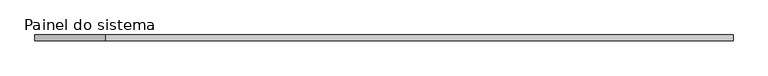
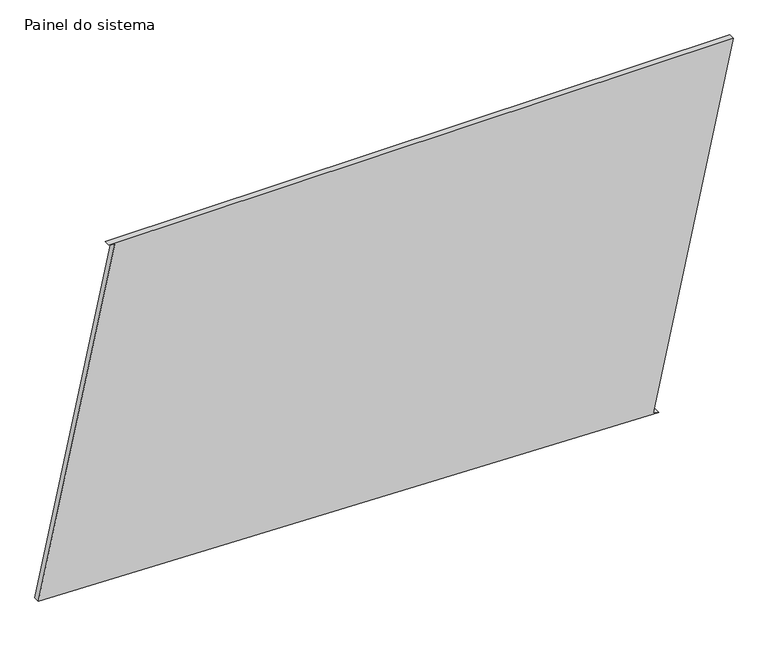
"""IFC4 building model written with IfcOpenShell, lengths in millimetres: plate geometry, Painel do sistema : Envidraçado."""

import ifcopenshell
import ifcopenshell.guid

model = None  # the IFC model being written
_history = None  # IfcOwnerHistory: only IFC2X3 demands one
_inside = {}  # id of a spatial element -> (the spatial element, [elements in it])
_under = {}  # id of a project, library or spatial element -> (it, [spatial elements below it])
_declared = {}  # id of a project -> (the project, [libraries it declares])
_typed = {}  # id of a type object -> (the type object, [elements of that type])
_made_of = {}  # id of a material, layer set ... -> (it, [elements and type objects made of it])


def new_model(schema):
    """Start an empty IFC model of exactly this schema.

    Asked for "IFC4X3", IfcOpenShell would pick the latest addendum, in which some entities
    have other attributes; the version numbers below select the first issue.
    IFC2X3 requires an IfcOwnerHistory on every rooted entity: one is made here for all.
    """
    global model, _history
    if schema == "IFC4X3":
        model = ifcopenshell.file(schema_version=(4, 3, 0, 0))
    else:
        model = ifcopenshell.file(schema=schema)
    _inside.clear()
    _under.clear()
    _declared.clear()
    _typed.clear()
    _made_of.clear()
    _history = None
    if model.schema == "IFC2X3":
        org = make("IfcOrganization", Name="unknown")
        user = make(
            "IfcPersonAndOrganization",
            ThePerson=make("IfcPerson", FamilyName="unknown"),
            TheOrganization=org,
        )
        app = make(
            "IfcApplication",
            ApplicationDeveloper=org,
            Version="unknown",
            ApplicationFullName="unknown",
            ApplicationIdentifier="unknown",
        )
        _history = make(
            "IfcOwnerHistory",
            OwningUser=user,
            OwningApplication=app,
            ChangeAction="ADDED",
            CreationDate=0,
        )
    return model


def make(cls, **values):
    """One entity of the class cls with the attributes given. An attribute that is None is left unset."""
    return model.create_entity(
        cls, **{name: value for name, value in values.items() if value is not None}
    )


def rooted(cls, **values):
    """An entity with a GlobalId (a new one), such as an element, a storey or a relation."""
    return make(cls, GlobalId=ifcopenshell.guid.new(), OwnerHistory=_history, **values)


def si_unit(unit_type, name, prefix=None):
    """IfcSIUnit, for example si_unit("LENGTHUNIT", "METRE", prefix="MILLI")."""
    return make("IfcSIUnit", UnitType=unit_type, Prefix=prefix, Name=name)


def assignment(units):
    """IfcUnitAssignment: the units of a project."""
    return None if units is None else make("IfcUnitAssignment", Units=units)


def point(xyz):
    """IfcCartesianPoint."""
    return None if xyz is None else make("IfcCartesianPoint", Coordinates=xyz)


def direction(xyz):
    """IfcDirection."""
    return None if xyz is None else make("IfcDirection", DirectionRatios=xyz)


def frame(location, z_axis=None, x_axis=None):
    """IfcAxis2Placement3D, a coordinate frame: its origin and axes. An axis left out is left unset."""
    return make(
        "IfcAxis2Placement3D",
        Location=point(location),
        Axis=direction(z_axis),
        RefDirection=direction(x_axis),
    )


def origin():
    """The frame at (0, 0, 0) with its axes left unset."""
    return frame((0.0, 0.0, 0.0))


def place(relative_to, where):
    """IfcLocalPlacement: puts the frame where relative to a parent placement (None: the world)."""
    return make(
        "IfcLocalPlacement", PlacementRelTo=relative_to, RelativePlacement=where
    )


def context(
    kind, dimensions, precision=None, world=None, true_north=None, identifier=None
):
    """IfcGeometricRepresentationContext, for example the 3D "Model" context."""
    return make(
        "IfcGeometricRepresentationContext",
        ContextIdentifier=identifier,
        ContextType=kind,
        CoordinateSpaceDimension=dimensions,
        Precision=precision,
        WorldCoordinateSystem=world,
        TrueNorth=true_north,
    )


def project(units=None, contexts=None):
    """IfcProject with its units and contexts."""
    return rooted(
        "IfcProject",
        Name="project",
        RepresentationContexts=contexts,
        UnitsInContext=assignment(units),
    )


def spatial(cls, under=None, at=None, **own):
    """A site, building, storey or space (cls), placed at a placement, below another one or the project."""
    s = rooted(cls, ObjectPlacement=at, **own)
    if under is not None:
        _under.setdefault(under.id(), (under, []))[1].append(s)
    return s


def polyline(points):
    """IfcPolyline through the points."""
    return make("IfcPolyline", Points=[point(p) for p in points])


def outline(outer, holes=None, kind="AREA"):
    """IfcArbitraryClosedProfileDef: a profile drawn as a closed curve; with holes, ...WithVoids."""
    if holes is None:
        return make("IfcArbitraryClosedProfileDef", ProfileType=kind, OuterCurve=outer)
    return make(
        "IfcArbitraryProfileDefWithVoids",
        ProfileType=kind,
        OuterCurve=outer,
        InnerCurves=holes,
    )


def extrude(swept, where, along, depth):
    """IfcExtrudedAreaSolid: the profile swept, set in the frame where, extruded along a direction by depth."""
    return make(
        "IfcExtrudedAreaSolid",
        SweptArea=swept,
        Position=where,
        ExtrudedDirection=direction(along),
        Depth=depth,
    )


def shape(context_of_items, identifier, shape_type, items):
    """IfcShapeRepresentation: the items that make up one representation, for example the "Body"."""
    return make(
        "IfcShapeRepresentation",
        ContextOfItems=context_of_items,
        RepresentationIdentifier=identifier,
        RepresentationType=shape_type,
        Items=items,
    )


def source(mapping_origin, context_of_items, identifier, shape_type, items):
    """IfcRepresentationMap: a shape defined once, which mapped items show again and again."""
    return make(
        "IfcRepresentationMap",
        MappingOrigin=mapping_origin,
        MappedRepresentation=shape(context_of_items, identifier, shape_type, items),
    )


def transform(
    local_origin,
    x_axis=None,
    y_axis=None,
    z_axis=None,
    scale=None,
    scale2=None,
    scale3=None,
    uniform=True,
):
    """IfcCartesianTransformationOperator3D, or its non-uniform kind. x_axis, y_axis, z_axis: its Axis1, 2, 3."""
    if uniform:
        return make(
            "IfcCartesianTransformationOperator3D",
            Axis1=direction(x_axis),
            Axis2=direction(y_axis),
            LocalOrigin=point(local_origin),
            Scale=scale,
            Axis3=direction(z_axis),
        )
    return make(
        "IfcCartesianTransformationOperator3DnonUniform",
        Axis1=direction(x_axis),
        Axis2=direction(y_axis),
        LocalOrigin=point(local_origin),
        Scale=scale,
        Axis3=direction(z_axis),
        Scale2=scale2,
        Scale3=scale3,
    )


def mapped(mapping_source, mapping_target):
    """IfcMappedItem: shows the shape of a source again, moved by a transform."""
    return make(
        "IfcMappedItem", MappingSource=mapping_source, MappingTarget=mapping_target
    )


def made_of(thing, what):
    """Note that an element or type object is made of a material, layer set ...; save() writes the relation."""
    if what is not None:
        _made_of.setdefault(what.id(), (what, []))[1].append(thing)
    return thing


def element(
    cls,
    number,
    at=None,
    inside=None,
    cuts=None,
    type_object=None,
    material=None,
    context=None,
    identifier="Body",
    shape_type=None,
    held_by="IfcProductDefinitionShape",
    body=None,
    shapes=None,
    **own,
):
    """One element of the class cls, such as IfcWall. Its Tag is "e" and its number.

    at: its placement. inside: the storey or other place that contains it. cuts: it is an
    opening in that element (IfcRelVoidsElement). A single representation is given by context,
    identifier, shape_type and body (its items); several are given by shapes. held_by: the class
    of the entity that holds the representations. save() writes the other relations.
    """
    e = rooted(cls, Tag="e%d" % number, ObjectPlacement=at, **own)
    if body is not None:
        shapes = [shape(context, identifier, shape_type, body)]
    if shapes is not None:
        e.Representation = make(held_by, Representations=shapes)
    if inside is not None:
        _inside.setdefault(inside.id(), (inside, []))[1].append(e)
    if cuts is not None:
        rooted(
            "IfcRelVoidsElement", RelatingBuildingElement=cuts, RelatedOpeningElement=e
        )
    if type_object is not None:
        _typed.setdefault(type_object.id(), (type_object, []))[1].append(e)
    return made_of(e, material)


def aggregate(whole, parts):
    """IfcRelAggregates: a whole, such as a stair, and the parts it consists of."""
    return rooted("IfcRelAggregates", RelatingObject=whole, RelatedObjects=parts)


def save(model, path):
    """Write the relations noted so far, then the file.

    IfcRelAggregates (storeys below a building ...), IfcRelContainedInSpatialStructure (elements
    in a storey), IfcRelDefinesByType, IfcRelAssociatesMaterial and IfcRelDeclares: one each for
    every whole, place, type object, material and project.
    """
    for whole, parts in _under.values():
        aggregate(whole, parts)
    for where, things in _inside.values():
        rooted(
            "IfcRelContainedInSpatialStructure",
            RelatedElements=things,
            RelatingStructure=where,
        )
    for kind, things in _typed.values():
        rooted("IfcRelDefinesByType", RelatedObjects=things, RelatingType=kind)
    for what, things in _made_of.values():
        rooted("IfcRelAssociatesMaterial", RelatedObjects=things, RelatingMaterial=what)
    for by, libraries in _declared.values():
        rooted("IfcRelDeclares", RelatingContext=by, RelatedDefinitions=libraries)
    model.write(path)


def painel_do_sistema_c43843b5(model_context):
    return source(origin(), model_context, "Body", "SweptSolid", [
        extrude(outline(polyline([(0.0, 1140.6960086), (5.3087357, 1116.2661637), (1544.5837464, 1450.7588362), (1544.5837464, -1156.3278443), (1539.2750108, -1131.8979993), (71.9348913, -1450.7588362), (0.0, 1140.6960086)])), frame((0.0, 24.5, 0.0), z_axis=(0.0, 1.0, 0.0), x_axis=(0.0, 0.0, 1.0)), (0.0, 0.0, 1.0), 25.0),
    ])


if __name__ == "__main__":
    model = new_model("IFC4")
    model_context = context("Model", 3, world=origin())
    ifc_project = project(units=[si_unit("LENGTHUNIT", "METRE", prefix="MILLI")], contexts=[model_context])
    site = spatial("IfcSite", under=ifc_project)
    building = spatial("IfcBuilding", under=site)
    placement = place(None, origin())
    painel_do_sistema_shape = painel_do_sistema_c43843b5(model_context)
    element("IfcPlate", 1, ObjectType="Painel do sistema : Envidraçado", at=placement, inside=building, context=model_context, shape_type="MappedRepresentation", body=[
        mapped(painel_do_sistema_shape, transform((0.0, 0.0, 0.0), x_axis=(1.0, 0.0, 0.0), y_axis=(0.0, 1.0, 0.0), z_axis=(0.0, 0.0, 1.0))),
    ])
    save(model, "model.ifc")

# Revit data of these elements
# Type "Painel do sistema : Envidraçado"
#   Construction Type Id = "GSP4R"
#   Analytic Construction = "Vidraça única Pilkington 1/8 pol"
#   Visual Light Transmittance = 0.9
#   Solar Heat Gain Coefficient = 0.86
#   Heat Transfer Coefficient (U) = 6.7069 W/(m²·K)
# Element 1 (IfcPlate, "Painel do sistema : Envidraçado")
#   Materials on its faces: "Vidro"
# Materials
#   "Vidro": class "Vidro", colour RGB 0 128 192, transparency 0.9, Description = "Vidro de sílica", Cost = 0
